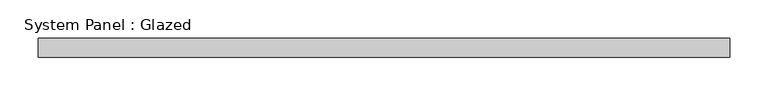
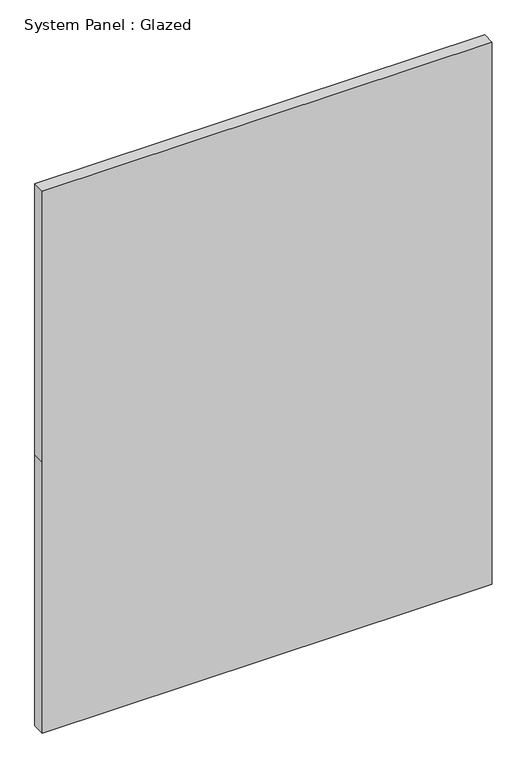
"""IFC4 building model written with IfcOpenShell, lengths in millimetres: plate geometry, System Panel : Glazed."""

import ifcopenshell
import ifcopenshell.guid

model = None  # the IFC model being written
_history = None  # IfcOwnerHistory: only IFC2X3 demands one
_inside = {}  # id of a spatial element -> (the spatial element, [elements in it])
_under = {}  # id of a project, library or spatial element -> (it, [spatial elements below it])
_declared = {}  # id of a project -> (the project, [libraries it declares])
_typed = {}  # id of a type object -> (the type object, [elements of that type])
_made_of = {}  # id of a material, layer set ... -> (it, [elements and type objects made of it])


def new_model(schema):
    """Start an empty IFC model of exactly this schema.

    Asked for "IFC4X3", IfcOpenShell would pick the latest addendum, in which some entities
    have other attributes; the version numbers below select the first issue.
    IFC2X3 requires an IfcOwnerHistory on every rooted entity: one is made here for all.
    """
    global model, _history
    if schema == "IFC4X3":
        model = ifcopenshell.file(schema_version=(4, 3, 0, 0))
    else:
        model = ifcopenshell.file(schema=schema)
    _inside.clear()
    _under.clear()
    _declared.clear()
    _typed.clear()
    _made_of.clear()
    _history = None
    if model.schema == "IFC2X3":
        org = make("IfcOrganization", Name="unknown")
        user = make(
            "IfcPersonAndOrganization",
            ThePerson=make("IfcPerson", FamilyName="unknown"),
            TheOrganization=org,
        )
        app = make(
            "IfcApplication",
            ApplicationDeveloper=org,
            Version="unknown",
            ApplicationFullName="unknown",
            ApplicationIdentifier="unknown",
        )
        _history = make(
            "IfcOwnerHistory",
            OwningUser=user,
            OwningApplication=app,
            ChangeAction="ADDED",
            CreationDate=0,
        )
    return model


def make(cls, **values):
    """One entity of the class cls with the attributes given. An attribute that is None is left unset."""
    return model.create_entity(
        cls, **{name: value for name, value in values.items() if value is not None}
    )


def rooted(cls, **values):
    """An entity with a GlobalId (a new one), such as an element, a storey or a relation."""
    return make(cls, GlobalId=ifcopenshell.guid.new(), OwnerHistory=_history, **values)


def si_unit(unit_type, name, prefix=None):
    """IfcSIUnit, for example si_unit("LENGTHUNIT", "METRE", prefix="MILLI")."""
    return make("IfcSIUnit", UnitType=unit_type, Prefix=prefix, Name=name)


def assignment(units):
    """IfcUnitAssignment: the units of a project."""
    return None if units is None else make("IfcUnitAssignment", Units=units)


def point(xyz):
    """IfcCartesianPoint."""
    return None if xyz is None else make("IfcCartesianPoint", Coordinates=xyz)


def direction(xyz):
    """IfcDirection."""
    return None if xyz is None else make("IfcDirection", DirectionRatios=xyz)


def frame(location, z_axis=None, x_axis=None):
    """IfcAxis2Placement3D, a coordinate frame: its origin and axes. An axis left out is left unset."""
    return make(
        "IfcAxis2Placement3D",
        Location=point(location),
        Axis=direction(z_axis),
        RefDirection=direction(x_axis),
    )


def origin():
    """The frame at (0, 0, 0) with its axes left unset."""
    return frame((0.0, 0.0, 0.0))


def place(relative_to, where):
    """IfcLocalPlacement: puts the frame where relative to a parent placement (None: the world)."""
    return make(
        "IfcLocalPlacement", PlacementRelTo=relative_to, RelativePlacement=where
    )


def context(
    kind, dimensions, precision=None, world=None, true_north=None, identifier=None
):
    """IfcGeometricRepresentationContext, for example the 3D "Model" context."""
    return make(
        "IfcGeometricRepresentationContext",
        ContextIdentifier=identifier,
        ContextType=kind,
        CoordinateSpaceDimension=dimensions,
        Precision=precision,
        WorldCoordinateSystem=world,
        TrueNorth=true_north,
    )


def project(units=None, contexts=None):
    """IfcProject with its units and contexts."""
    return rooted(
        "IfcProject",
        Name="project",
        RepresentationContexts=contexts,
        UnitsInContext=assignment(units),
    )


def spatial(cls, under=None, at=None, **own):
    """A site, building, storey or space (cls), placed at a placement, below another one or the project."""
    s = rooted(cls, ObjectPlacement=at, **own)
    if under is not None:
        _under.setdefault(under.id(), (under, []))[1].append(s)
    return s


def polyline(points):
    """IfcPolyline through the points."""
    return make("IfcPolyline", Points=[point(p) for p in points])


def outline(outer, holes=None, kind="AREA"):
    """IfcArbitraryClosedProfileDef: a profile drawn as a closed curve; with holes, ...WithVoids."""
    if holes is None:
        return make("IfcArbitraryClosedProfileDef", ProfileType=kind, OuterCurve=outer)
    return make(
        "IfcArbitraryProfileDefWithVoids",
        ProfileType=kind,
        OuterCurve=outer,
        InnerCurves=holes,
    )


def extrude(swept, where, along, depth):
    """IfcExtrudedAreaSolid: the profile swept, set in the frame where, extruded along a direction by depth."""
    return make(
        "IfcExtrudedAreaSolid",
        SweptArea=swept,
        Position=where,
        ExtrudedDirection=direction(along),
        Depth=depth,
    )


def shape(context_of_items, identifier, shape_type, items):
    """IfcShapeRepresentation: the items that make up one representation, for example the "Body"."""
    return make(
        "IfcShapeRepresentation",
        ContextOfItems=context_of_items,
        RepresentationIdentifier=identifier,
        RepresentationType=shape_type,
        Items=items,
    )


def source(mapping_origin, context_of_items, identifier, shape_type, items):
    """IfcRepresentationMap: a shape defined once, which mapped items show again and again."""
    return make(
        "IfcRepresentationMap",
        MappingOrigin=mapping_origin,
        MappedRepresentation=shape(context_of_items, identifier, shape_type, items),
    )


def transform(
    local_origin,
    x_axis=None,
    y_axis=None,
    z_axis=None,
    scale=None,
    scale2=None,
    scale3=None,
    uniform=True,
):
    """IfcCartesianTransformationOperator3D, or its non-uniform kind. x_axis, y_axis, z_axis: its Axis1, 2, 3."""
    if uniform:
        return make(
            "IfcCartesianTransformationOperator3D",
            Axis1=direction(x_axis),
            Axis2=direction(y_axis),
            LocalOrigin=point(local_origin),
            Scale=scale,
            Axis3=direction(z_axis),
        )
    return make(
        "IfcCartesianTransformationOperator3DnonUniform",
        Axis1=direction(x_axis),
        Axis2=direction(y_axis),
        LocalOrigin=point(local_origin),
        Scale=scale,
        Axis3=direction(z_axis),
        Scale2=scale2,
        Scale3=scale3,
    )


def mapped(mapping_source, mapping_target):
    """IfcMappedItem: shows the shape of a source again, moved by a transform."""
    return make(
        "IfcMappedItem", MappingSource=mapping_source, MappingTarget=mapping_target
    )


def made_of(thing, what):
    """Note that an element or type object is made of a material, layer set ...; save() writes the relation."""
    if what is not None:
        _made_of.setdefault(what.id(), (what, []))[1].append(thing)
    return thing


def element(
    cls,
    number,
    at=None,
    inside=None,
    cuts=None,
    type_object=None,
    material=None,
    context=None,
    identifier="Body",
    shape_type=None,
    held_by="IfcProductDefinitionShape",
    body=None,
    shapes=None,
    **own,
):
    """One element of the class cls, such as IfcWall. Its Tag is "e" and its number.

    at: its placement. inside: the storey or other place that contains it. cuts: it is an
    opening in that element (IfcRelVoidsElement). A single representation is given by context,
    identifier, shape_type and body (its items); several are given by shapes. held_by: the class
    of the entity that holds the representations. save() writes the other relations.
    """
    e = rooted(cls, Tag="e%d" % number, ObjectPlacement=at, **own)
    if body is not None:
        shapes = [shape(context, identifier, shape_type, body)]
    if shapes is not None:
        e.Representation = make(held_by, Representations=shapes)
    if inside is not None:
        _inside.setdefault(inside.id(), (inside, []))[1].append(e)
    if cuts is not None:
        rooted(
            "IfcRelVoidsElement", RelatingBuildingElement=cuts, RelatedOpeningElement=e
        )
    if type_object is not None:
        _typed.setdefault(type_object.id(), (type_object, []))[1].append(e)
    return made_of(e, material)


def aggregate(whole, parts):
    """IfcRelAggregates: a whole, such as a stair, and the parts it consists of."""
    return rooted("IfcRelAggregates", RelatingObject=whole, RelatedObjects=parts)


def save(model, path):
    """Write the relations noted so far, then the file.

    IfcRelAggregates (storeys below a building ...), IfcRelContainedInSpatialStructure (elements
    in a storey), IfcRelDefinesByType, IfcRelAssociatesMaterial and IfcRelDeclares: one each for
    every whole, place, type object, material and project.
    """
    for whole, parts in _under.values():
        aggregate(whole, parts)
    for where, things in _inside.values():
        rooted(
            "IfcRelContainedInSpatialStructure",
            RelatedElements=things,
            RelatingStructure=where,
        )
    for kind, things in _typed.values():
        rooted("IfcRelDefinesByType", RelatedObjects=things, RelatingType=kind)
    for what, things in _made_of.values():
        rooted("IfcRelAssociatesMaterial", RelatedObjects=things, RelatingMaterial=what)
    for by, libraries in _declared.values():
        rooted("IfcRelDeclares", RelatingContext=by, RelatedDefinitions=libraries)
    model.write(path)


def system_panel_glazed_44d19d28(model_context):
    return source(origin(), model_context, "Body", "SweptSolid", [
        extrude(outline(polyline([(0.0, -454.025), (0.0, 454.025), (577.85, 454.025), (1155.7, 454.025), (1155.7, -454.025), (577.85, -454.025), (0.0, -454.025)])), frame((0.0, -44.45, 0.0), z_axis=(0.0, 1.0, 0.0), x_axis=(0.0, 0.0, 1.0)), (0.0, 0.0, 1.0), 25.4),
    ])


if __name__ == "__main__":
    model = new_model("IFC4")
    model_context = context("Model", 3, world=origin())
    ifc_project = project(units=[si_unit("LENGTHUNIT", "METRE", prefix="MILLI")], contexts=[model_context])
    site = spatial("IfcSite", under=ifc_project)
    building = spatial("IfcBuilding", under=site)
    placement = place(None, origin())
    system_panel_glazed_shape = system_panel_glazed_44d19d28(model_context)
    element("IfcPlate", 1, ObjectType="System Panel : Glazed", at=placement, inside=building, context=model_context, shape_type="MappedRepresentation", body=[
        mapped(system_panel_glazed_shape, transform((0.0, 0.0, 0.0), x_axis=(1.0, 0.0, 0.0), y_axis=(0.0, 1.0, 0.0), z_axis=(0.0, 0.0, 1.0))),
    ])
    save(model, "model.ifc")

# Revit data of these elements
# Element 1 (IfcPlate, "System Panel : Glazed")
#   Materials on its faces: "Glass"
# Materials
#   "Glass": class "Unassigned", colour RGB 0 0 255, transparency 0.75
